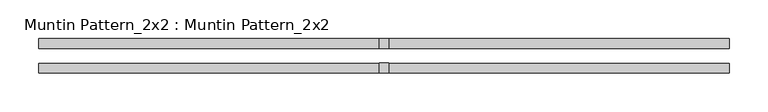
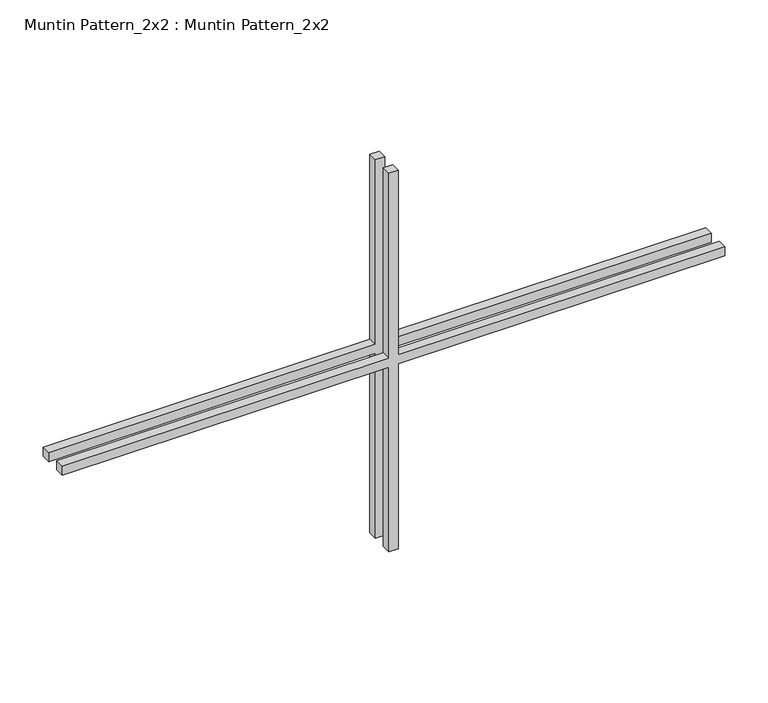
"""IFC4 building model written with IfcOpenShell, lengths in millimetres: proxy geometry, Muntin Pattern_2x2 : Muntin Pattern_2x2."""

from ifc_helpers import new_model, si_unit, frame, origin, place, context, project, spatial, polyline, outline, extrude, source, transform, mapped, element, save


def muntin_pattern_2x2_muntin_pattern_2x2_50d3873d(model_context):
    return source(origin(), model_context, "Body", "SweptSolid", [
        extrude(outline(polyline([(274.6375, -6.35), (274.6375, -444.5), (261.9375, -444.5), (261.9375, -6.35), (0.0, -6.35), (0.0, 6.35), (261.9375, 6.35), (261.9375, 444.5), (274.6375, 444.5), (274.6375, 6.35), (536.575, 6.35), (536.575, -6.35), (274.6375, -6.35)])), frame((0.0, -22.225, 0.0), z_axis=(0.0, 1.0, 0.0), x_axis=(0.0, 0.0, 1.0)), (0.0, 0.0, 1.0), 12.7),
        extrude(outline(polyline([(274.6375, -6.35), (274.6375, -444.5), (261.9375, -444.5), (261.9375, -6.35), (0.0, -6.35), (0.0, 6.35), (261.9375, 6.35), (261.9375, 444.5), (274.6375, 444.5), (274.6375, 6.35), (536.575, 6.35), (536.575, -6.35), (274.6375, -6.35)])), frame((0.0, 9.525, 0.0), z_axis=(0.0, 1.0, 0.0), x_axis=(0.0, 0.0, 1.0)), (0.0, 0.0, 1.0), 12.7),
    ])


if __name__ == "__main__":
    model = new_model("IFC4")
    model_context = context("Model", 3, world=origin())
    ifc_project = project(units=[si_unit("LENGTHUNIT", "METRE", prefix="MILLI")], contexts=[model_context])
    site = spatial("IfcSite", under=ifc_project)
    building = spatial("IfcBuilding", under=site)
    placement = place(None, origin())
    muntin_pattern_2x2_muntin_pattern_2x2_shape = muntin_pattern_2x2_muntin_pattern_2x2_50d3873d(model_context)
    element("IfcBuildingElementProxy", 1, Name="Muntin Pattern_2x2 : Muntin Pattern_2x2", ObjectType="Muntin Pattern_2x2 : Muntin Pattern_2x2", at=placement, inside=building, context=model_context, shape_type="MappedRepresentation", body=[
        mapped(muntin_pattern_2x2_muntin_pattern_2x2_shape, transform((0.0, 0.0, 0.0), x_axis=(1.0, 0.0, 0.0), y_axis=(0.0, 1.0, 0.0), z_axis=(0.0, 0.0, 1.0))),
    ])
    save(model, "model.ifc")

# Revit data of these elements
# Type "Muntin Pattern_2x2 : Muntin Pattern_2x2"
#   Width [instance default] = 4' - 0"
#   Thickness = 0' - 0 1/2"
#   Height [instance default] = 4' - 0"
#   Distance = 0' - 0 3/4"
#   Interior Material [instance default] = none
#   Exterior Material [instance default] = none
# Element 1 (IfcBuildingElementProxy, "Muntin Pattern_2x2 : Muntin Pattern_2x2")
#   Width = 2' - 11"
#   Height = 1' - 9 1/8"
#   Interior Material = Wood - Stained
#   Exterior Material = Clad - White
#   Materials on its faces: "Clad - White", "Wood - Stained"
# Materials
#   "Clad - White": class "Wood", colour RGB 242 242 238, transparency 0, Cost = 0
#   "Wood - Stained": class "Wood", colour RGB 224 178 126, transparency 0, Cost = 0
